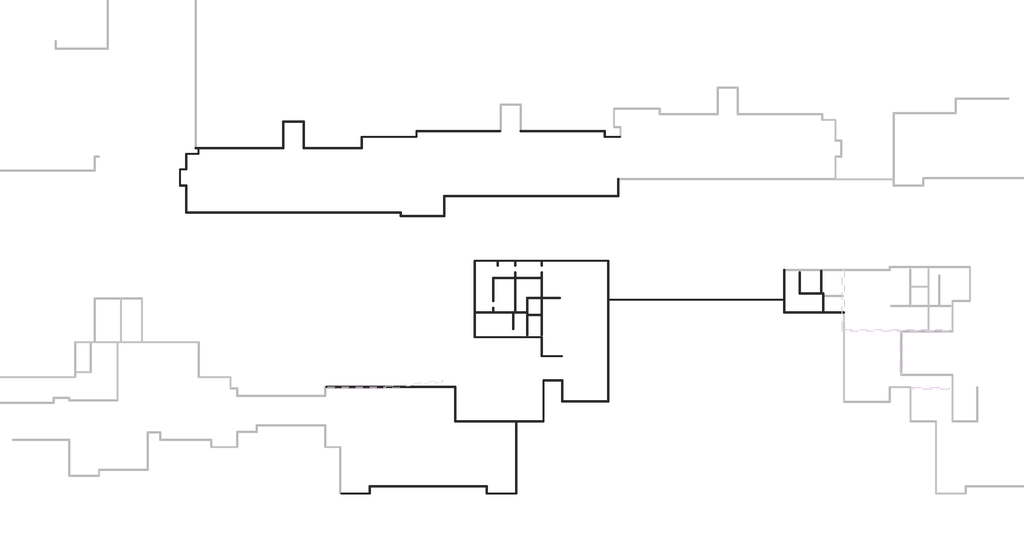
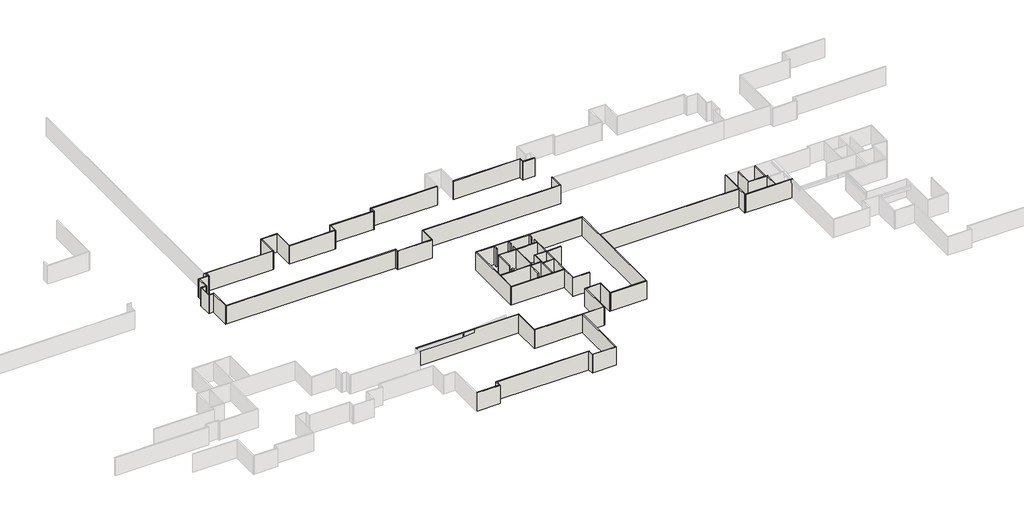
# One storey, part 4 of 8: 65 walls.
"""IFC4 building model written with IfcOpenShell, lengths in millimetres."""

from ifc_helpers import new_model, si_unit, origin, origin_with_axes, place, context, project, spatial, polyline, outline, extrude, faceted_brep, element, save

model = new_model("IFC4")

# Units and contexts
model_context = context("Model", 3, world=origin())
ifc_project = project(units=[si_unit("LENGTHUNIT", "METRE", prefix="MILLI")], contexts=[model_context])

# Site, building, storey
site = spatial("IfcSite", under=ifc_project)
building = spatial("IfcBuilding", under=site)
storey = spatial("IfcBuildingStorey", under=building, Name="户型图", Elevation=0.0)

# Walls
placement = place(None, origin())
element("IfcWall", 1, ObjectType="所有墙体", at=placement, inside=storey, context=model_context, shape_type="Brep", body=[
    faceted_brep([(190584.1761986, 13145.7645172, 0.0), (194584.1250491, 13145.7645172, 0.0), (194584.1250491, 13145.7645172, 3300.0), (190584.1761986, 13145.7645172, 3300.0), (190584.1761986, 13265.7645172, 0.0), (190584.1761986, 13265.7645172, 3300.0), (194464.1250491, 13265.7645172, 3300.0), (194584.1250491, 13265.7645172, 3300.0), (194584.1250491, 13265.7645172, 0.0), (194464.1250491, 13265.7645172, 0.0)], [[[0, 1, 2, 3]], [[4, 5, 6, 7, 8, 9]], [[1, 0, 4, 9, 8]], [[3, 2, 7, 6, 5]], [[0, 3, 5, 4]], [[2, 1, 8, 7]]]),
])
element("IfcWall", 2, ObjectType="所有墙体", at=placement, inside=storey, context=model_context, shape_type="Brep", body=[
    faceted_brep([(194584.1250491, 13265.7645172, 0.0), (194584.1250491, 14145.6242927, 0.0), (194584.1250491, 14265.6242927, 0.0), (194584.1250491, 14265.6242927, 3300.0), (194584.1250491, 14145.6242927, 3300.0), (194584.1250491, 13265.7645172, 3300.0), (194464.1250491, 13265.7645172, 0.0), (194464.1250491, 13265.7645172, 3300.0), (194464.1250491, 14265.6242927, 3300.0), (194464.1250491, 14265.6242927, 0.0)], [[[0, 1, 2, 3, 4, 5]], [[6, 7, 8, 9]], [[2, 1, 0, 6, 9]], [[5, 4, 3, 8, 7]], [[0, 5, 7, 6]], [[3, 2, 9, 8]]]),
])
element("IfcWall", 3, ObjectType="所有墙体", at=placement, inside=storey, context=model_context, shape_type="Brep", body=[
    faceted_brep([(194584.1250491, 14145.6242927, 0.0), (210264.1178879, 14145.6242927, 0.0), (210384.1178879, 14145.6242927, 0.0), (210384.1178879, 14145.6242927, 3300.0), (210264.1178879, 14145.6242927, 3300.0), (194584.1250491, 14145.6242927, 3300.0), (194584.1250491, 14265.6242927, 0.0), (194584.1250491, 14265.6242927, 3300.0), (210384.1178879, 14265.6242927, 3300.0), (210384.1178879, 14265.6242927, 0.0)], [[[0, 1, 2, 3, 4, 5]], [[6, 7, 8, 9]], [[2, 1, 0, 6, 9]], [[5, 4, 3, 8, 7]], [[0, 5, 7, 6]], [[3, 2, 9, 8]]]),
])
element("IfcWall", 4, ObjectType="所有墙体", at=placement, inside=storey, context=model_context, shape_type="Brep", body=[
    faceted_brep([(210264.1178879, 14145.6242927, 0.0), (210264.1178879, 13145.7645172, 0.0), (210264.1178879, 13145.7645172, 3300.0), (210264.1178879, 14145.6242927, 3300.0), (210384.1178879, 14145.6242927, 0.0), (210384.1178879, 14145.6242927, 3300.0), (210384.1178879, 13265.7645172, 3300.0), (210384.1178879, 13145.7645172, 3300.0), (210384.1178879, 13145.7645172, 0.0), (210384.1178879, 13265.7645172, 0.0)], [[[0, 1, 2, 3]], [[4, 5, 6, 7, 8, 9]], [[1, 0, 4, 9, 8]], [[3, 2, 7, 6, 5]], [[0, 3, 5, 4]], [[2, 1, 8, 7]]]),
])
element("IfcWall", 5, ObjectType="所有墙体", at=placement, inside=storey, context=model_context, shape_type="Brep", body=[
    faceted_brep([(210384.1178879, 13145.7645172, 0.0), (214384.1922923, 13145.7645172, 0.0), (214384.1922923, 13145.7645172, 3300.0), (210384.1178879, 13145.7645172, 3300.0), (210384.1178879, 13265.7645172, 0.0), (210384.1178879, 13265.7645172, 3300.0), (214264.1922923, 13265.7645172, 3300.0), (214384.1922923, 13265.7645172, 3300.0), (214384.1922923, 13265.7645172, 0.0), (214264.1922923, 13265.7645172, 0.0)], [[[0, 1, 2, 3]], [[4, 5, 6, 7, 8, 9]], [[1, 0, 4, 9, 8]], [[3, 2, 7, 6, 5]], [[0, 3, 5, 4]], [[2, 1, 8, 7]]]),
])
element("IfcWall", 6, ObjectType="所有墙体", at=placement, inside=storey, context=model_context, shape_type="SweptSolid", body=[
    extrude(outline(polyline([(214384.1922923, 22945.5527507), (214384.1922923, 13265.7645172), (214264.1922923, 13265.7645172), (214264.1922923, 22945.5527507), (214384.1922923, 22945.5527507)])), origin_with_axes(), (0.0, 0.0, 1.0), 3300.0),
])
element("IfcWall", 7, ObjectType="所有墙体", at=placement, inside=storey, context=model_context, shape_type="Brep", body=[
    faceted_brep([(218064.1922923, 22945.5527507, 0.0), (218064.1922923, 28456.6703435, 0.0), (218064.1922923, 28576.6703435, 0.0), (218064.1922923, 28576.6703435, 3300.0), (218064.1922923, 28456.6703435, 3300.0), (218064.1922923, 22945.5527507, 3300.0), (217944.1922923, 22945.5527507, 0.0), (217944.1922923, 22945.5527507, 3300.0), (217944.1922923, 23065.5527507, 3300.0), (217944.1922923, 28576.6703435, 3300.0), (217944.1922923, 28576.6703435, 0.0), (217944.1922923, 23065.5527507, 0.0)], [[[0, 1, 2, 3, 4, 5]], [[6, 7, 8, 9, 10, 11]], [[2, 1, 0, 6, 11, 10]], [[5, 4, 3, 9, 8, 7]], [[3, 2, 10, 9]], [[0, 5, 7, 6]]]),
])
element("IfcWall", 8, ObjectType="所有墙体", at=placement, inside=storey, context=model_context, shape_type="Brep", body=[
    faceted_brep([(218064.1922923, 28456.6703435, 0.0), (220514.3505603, 28456.6703435, 0.0), (220634.3505603, 28456.6703435, 0.0), (220634.3505603, 28456.6703435, 3300.0), (220514.3505603, 28456.6703435, 3300.0), (218064.1922923, 28456.6703435, 3300.0), (218064.1922923, 28576.6703435, 0.0), (218064.1922923, 28576.6703435, 3300.0), (220634.3505603, 28576.6703435, 3300.0), (220634.3505603, 28576.6703435, 0.0)], [[[0, 1, 2, 3, 4, 5]], [[6, 7, 8, 9]], [[2, 1, 0, 6, 9]], [[5, 4, 3, 8, 7]], [[0, 5, 7, 6]], [[3, 2, 9, 8]]]),
])
element("IfcWall", 9, ObjectType="所有墙体", at=placement, inside=storey, context=model_context, shape_type="Brep", body=[
    faceted_brep([(220514.3505603, 28456.6703435, 0.0), (220514.3505603, 25645.6713095, 0.0), (220514.3505603, 25645.6713095, 3300.0), (220514.3505603, 28456.6703435, 3300.0), (220634.3505603, 28456.6703435, 0.0), (220634.3505603, 28456.6703435, 3300.0), (220634.3505603, 25765.6713095, 3300.0), (220634.3505603, 25645.6713095, 3300.0), (220634.3505603, 25645.6713095, 0.0), (220634.3505603, 25765.6713095, 0.0)], [[[0, 1, 2, 3]], [[4, 5, 6, 7, 8, 9]], [[1, 0, 4, 9, 8]], [[3, 2, 7, 6, 5]], [[0, 3, 5, 4]], [[2, 1, 8, 7]]]),
])
element("IfcWall", 10, ObjectType="所有墙体", at=placement, inside=storey, context=model_context, shape_type="Brep", body=[
    faceted_brep([(220634.3505603, 25645.6713095, 0.0), (226833.8525836, 25645.6713095, 0.0), (226833.8525836, 25645.6713095, 3300.0), (220634.3505603, 25645.6713095, 3300.0), (220634.3505603, 25765.6713095, 0.0), (220634.3505603, 25765.6713095, 3300.0), (226713.8525836, 25765.6713095, 3300.0), (226833.8525836, 25765.6713095, 3300.0), (226833.8525836, 25765.6713095, 0.0), (226713.8525836, 25765.6713095, 0.0)], [[[0, 1, 2, 3]], [[4, 5, 6, 7, 8, 9]], [[1, 0, 4, 9, 8]], [[3, 2, 7, 6, 5]], [[0, 3, 5, 4]], [[2, 1, 8, 7]]]),
])
element("IfcWall", 11, ObjectType="所有墙体", at=placement, inside=storey, context=model_context, shape_type="Brep", body=[
    faceted_brep([(226833.8525836, 25765.6713095, 0.0), (226833.8525836, 39406.3533948, 0.0), (226833.8525836, 39526.3533948, 0.0), (226833.8525836, 44681.8474602, 0.0), (226833.8525836, 44681.8474602, 3300.0), (226833.8525836, 39526.3533948, 3300.0), (226833.8525836, 39406.3533948, 3300.0), (226833.8525836, 25765.6713095, 3300.0), (226713.8525836, 25765.6713095, 0.0), (226713.8525836, 25765.6713095, 3300.0), (226713.8525836, 44681.8474602, 3300.0), (226713.8525836, 44681.8474602, 0.0)], [[[0, 1, 2, 3, 4, 5, 6, 7]], [[8, 9, 10, 11]], [[3, 2, 1, 0, 8, 11]], [[7, 6, 5, 4, 10, 9]], [[0, 7, 9, 8]], [[4, 3, 11, 10]]]),
])
element("IfcWall", 12, ObjectType="所有墙体", at=placement, inside=storey, context=model_context, shape_type="SweptSolid", body=[
    extrude(outline(polyline([(250538.8239575, 39406.3533948), (226833.8525836, 39406.3533948), (226833.8525836, 39526.3533948), (250538.8239575, 39526.3533948), (250538.8239575, 39406.3533948)])), origin_with_axes(), (0.0, 0.0, 1.0), 3300.0),
])
element("IfcWall", 13, ObjectType="所有墙体", at=placement, inside=storey, context=model_context, shape_type="Brep", body=[
    faceted_brep([(250538.8239575, 43526.8473728, 0.0), (250538.8239575, 39526.3533948, 0.0), (250538.8239575, 39406.3533948, 0.0), (250538.8239575, 37656.7427445, 0.0), (250538.8239575, 37656.7427445, 3300.0), (250538.8239575, 39406.3533948, 3300.0), (250538.8239575, 39526.3533948, 3300.0), (250538.8239575, 43526.8473728, 3300.0), (250658.8239575, 43526.8473728, 0.0), (250658.8239575, 43526.8473728, 3300.0), (250658.8239575, 43406.8473728, 3300.0), (250658.8239575, 37776.7427445, 3300.0), (250658.8239575, 37656.7427445, 3300.0), (250658.8239575, 37656.7427445, 0.0), (250658.8239575, 37776.7427445, 0.0), (250658.8239575, 43406.8473728, 0.0)], [[[0, 1, 2, 3, 4, 5, 6, 7]], [[8, 9, 10, 11, 12, 13, 14, 15]], [[3, 2, 1, 0, 8, 15, 14, 13]], [[7, 6, 5, 4, 12, 11, 10, 9]], [[4, 3, 13, 12]], [[0, 7, 9, 8]]]),
])
element("IfcWall", 14, ObjectType="所有墙体", at=placement, inside=storey, context=model_context, shape_type="Brep", body=[
    faceted_brep([(250658.8239575, 37656.7427445, 0.0), (258613.8534901, 37656.7427445, 0.0), (258733.8534901, 37656.7427445, 0.0), (258733.8534901, 37656.7427445, 3300.0), (258613.8534901, 37656.7427445, 3300.0), (250658.8239575, 37656.7427445, 3300.0), (250658.8239575, 37776.7427445, 0.0), (250658.8239575, 37776.7427445, 3300.0), (255788.6559976, 37776.7427445, 3300.0), (255908.6559976, 37776.7427445, 3300.0), (258733.8534901, 37776.7427445, 3300.0), (258733.8534901, 37776.7427445, 0.0), (255908.6559976, 37776.7427445, 0.0), (255788.6559976, 37776.7427445, 0.0)], [[[0, 1, 2, 3, 4, 5]], [[6, 7, 8, 9, 10, 11, 12, 13]], [[2, 1, 0, 6, 13, 12, 11]], [[5, 4, 3, 10, 9, 8, 7]], [[0, 5, 7, 6]], [[3, 2, 11, 10]]]),
])
element("IfcWall", 15, ObjectType="所有墙体", at=placement, inside=storey, context=model_context, shape_type="Brep", body=[
    faceted_brep([(228364.4881621, 61576.5107166, 0.0), (226384.4923674, 61576.5107166, 0.0), (226264.4923674, 61576.5107166, 0.0), (226264.4923674, 61576.5107166, 3300.0), (226384.4923674, 61576.5107166, 3300.0), (228364.4881621, 61576.5107166, 3300.0), (228364.4881621, 61456.5107166, 0.0), (228364.4881621, 61456.5107166, 3300.0), (226264.4923674, 61456.5107166, 3300.0), (226264.4923674, 61456.5107166, 0.0)], [[[0, 1, 2, 3, 4, 5]], [[6, 7, 8, 9]], [[2, 1, 0, 6, 9]], [[5, 4, 3, 8, 7]], [[0, 5, 7, 6]], [[3, 2, 9, 8]]]),
])
element("IfcWall", 16, ObjectType="所有墙体", at=placement, inside=storey, context=model_context, shape_type="Brep", body=[
    faceted_brep([(226384.4923674, 61576.5107166, 0.0), (226384.4923674, 62376.635741, 0.0), (226384.4923674, 62376.635741, 3300.0), (226384.4923674, 61576.5107166, 3300.0), (226264.4923674, 61576.5107166, 0.0), (226264.4923674, 61576.5107166, 3300.0), (226264.4923674, 62256.635741, 3300.0), (226264.4923674, 62376.635741, 3300.0), (226264.4923674, 62376.635741, 0.0), (226264.4923674, 62256.635741, 0.0)], [[[0, 1, 2, 3]], [[4, 5, 6, 7, 8, 9]], [[1, 0, 4, 9, 8]], [[3, 2, 7, 6, 5]], [[0, 3, 5, 4]], [[2, 1, 8, 7]]]),
])
element("IfcWall", 17, ObjectType="所有墙体", at=placement, inside=storey, context=model_context, shape_type="Brep", body=[
    faceted_brep([(226264.4923674, 62376.635741, 0.0), (214984.4914101, 62376.635741, 0.0), (214864.4914101, 62376.635741, 0.0), (214864.4914101, 62376.635741, 3300.0), (214984.4914101, 62376.635741, 3300.0), (226264.4923674, 62376.635741, 3300.0), (226264.4923674, 62256.635741, 0.0), (226264.4923674, 62256.635741, 3300.0), (214864.4914101, 62256.635741, 3300.0), (214864.4914101, 62256.635741, 0.0)], [[[0, 1, 2, 3, 4, 5]], [[6, 7, 8, 9]], [[2, 1, 0, 6, 9]], [[5, 4, 3, 8, 7]], [[0, 5, 7, 6]], [[3, 2, 9, 8]]]),
])
element("IfcWall", 18, ObjectType="所有墙体", at=placement, inside=storey, context=model_context, shape_type="Brep", body=[
    faceted_brep([(212164.4916662, 62376.635741, 0.0), (200764.4747442, 62376.635741, 0.0), (200764.4747442, 62376.635741, 3300.0), (212164.4916662, 62376.635741, 3300.0), (212164.4916662, 62256.635741, 0.0), (212164.4916662, 62256.635741, 3300.0), (200884.4747442, 62256.635741, 3300.0), (200764.4747442, 62256.635741, 3300.0), (200764.4747442, 62256.635741, 0.0), (200884.4747442, 62256.635741, 0.0)], [[[0, 1, 2, 3]], [[4, 5, 6, 7, 8, 9]], [[1, 0, 4, 9, 8]], [[3, 2, 7, 6, 5]], [[0, 3, 5, 4]], [[2, 1, 8, 7]]]),
])
element("IfcWall", 19, ObjectType="所有墙体", at=placement, inside=storey, context=model_context, shape_type="Brep", body=[
    faceted_brep([(200764.4747442, 62256.635741, 0.0), (200764.4747442, 61576.5107166, 0.0), (200764.4747442, 61456.5107166, 0.0), (200764.4747442, 61456.5107166, 3300.0), (200764.4747442, 61576.5107166, 3300.0), (200764.4747442, 62256.635741, 3300.0), (200884.4747442, 62256.635741, 0.0), (200884.4747442, 62256.635741, 3300.0), (200884.4747442, 61456.5107166, 3300.0), (200884.4747442, 61456.5107166, 0.0)], [[[0, 1, 2, 3, 4, 5]], [[6, 7, 8, 9]], [[2, 1, 0, 6, 9]], [[5, 4, 3, 8, 7]], [[0, 5, 7, 6]], [[3, 2, 9, 8]]]),
])
element("IfcWall", 20, ObjectType="所有墙体", at=placement, inside=storey, context=model_context, shape_type="Brep", body=[
    faceted_brep([(200764.4747442, 61576.5107166, 0.0), (193364.4739968, 61576.5107166, 0.0), (193364.4739968, 61576.5107166, 3300.0), (200764.4747442, 61576.5107166, 3300.0), (200764.4747442, 61456.5107166, 0.0), (200764.4747442, 61456.5107166, 3300.0), (193484.4739968, 61456.5107166, 3300.0), (193364.4739968, 61456.5107166, 3300.0), (193364.4739968, 61456.5107166, 0.0), (193484.4739968, 61456.5107166, 0.0)], [[[0, 1, 2, 3]], [[4, 5, 6, 7, 8, 9]], [[1, 0, 4, 9, 8]], [[3, 2, 7, 6, 5]], [[0, 3, 5, 4]], [[2, 1, 8, 7]]]),
])
element("IfcWall", 21, ObjectType="所有墙体", at=placement, inside=storey, context=model_context, shape_type="Brep", body=[
    faceted_brep([(193364.4739968, 61456.5107166, 0.0), (193364.4739968, 60076.635667, 0.0), (193364.4739968, 59956.635667, 0.0), (193364.4739968, 59956.635667, 3300.0), (193364.4739968, 60076.635667, 3300.0), (193364.4739968, 61456.5107166, 3300.0), (193484.4739968, 61456.5107166, 0.0), (193484.4739968, 61456.5107166, 3300.0), (193484.4739968, 59956.635667, 3300.0), (193484.4739968, 59956.635667, 0.0)], [[[0, 1, 2, 3, 4, 5]], [[6, 7, 8, 9]], [[2, 1, 0, 6, 9]], [[5, 4, 3, 8, 7]], [[0, 5, 7, 6]], [[3, 2, 9, 8]]]),
])
element("IfcWall", 22, ObjectType="所有墙体", at=placement, inside=storey, context=model_context, shape_type="Brep", body=[
    faceted_brep([(193364.4739968, 60076.635667, 0.0), (185609.4693749, 60076.635667, 0.0), (185489.4693749, 60076.635667, 0.0), (185489.4693749, 60076.635667, 3300.0), (185609.4693749, 60076.635667, 3300.0), (193364.4739968, 60076.635667, 3300.0), (193364.4739968, 59956.635667, 0.0), (193364.4739968, 59956.635667, 3300.0), (185489.4693749, 59956.635667, 3300.0), (185489.4693749, 59956.635667, 0.0)], [[[0, 1, 2, 3, 4, 5]], [[6, 7, 8, 9]], [[2, 1, 0, 6, 9]], [[5, 4, 3, 8, 7]], [[0, 5, 7, 6]], [[3, 2, 9, 8]]]),
])
element("IfcWall", 23, ObjectType="所有墙体", at=placement, inside=storey, context=model_context, shape_type="Brep", body=[
    faceted_brep([(185609.4693749, 60076.635667, 0.0), (185609.4693749, 63651.6355965, 0.0), (185609.4693749, 63651.6355965, 3300.0), (185609.4693749, 60076.635667, 3300.0), (185489.4693749, 60076.635667, 0.0), (185489.4693749, 60076.635667, 3300.0), (185489.4693749, 63531.6355965, 3300.0), (185489.4693749, 63651.6355965, 3300.0), (185489.4693749, 63651.6355965, 0.0), (185489.4693749, 63531.6355965, 0.0)], [[[0, 1, 2, 3]], [[4, 5, 6, 7, 8, 9]], [[1, 0, 4, 9, 8]], [[3, 2, 7, 6, 5]], [[0, 3, 5, 4]], [[2, 1, 8, 7]]]),
])
element("IfcWall", 24, ObjectType="所有墙体", at=placement, inside=storey, context=model_context, shape_type="Brep", body=[
    faceted_brep([(185489.4693749, 63651.6355965, 0.0), (182739.4693749, 63651.6355965, 0.0), (182739.4693749, 63651.6355965, 3300.0), (185489.4693749, 63651.6355965, 3300.0), (185489.4693749, 63531.6355965, 0.0), (185489.4693749, 63531.6355965, 3300.0), (182859.4693749, 63531.6355965, 3300.0), (182739.4693749, 63531.6355965, 3300.0), (182739.4693749, 63531.6355965, 0.0), (182859.4693749, 63531.6355965, 0.0)], [[[0, 1, 2, 3]], [[4, 5, 6, 7, 8, 9]], [[1, 0, 4, 9, 8]], [[3, 2, 7, 6, 5]], [[0, 3, 5, 4]], [[2, 1, 8, 7]]]),
])
element("IfcWall", 25, ObjectType="所有墙体", at=placement, inside=storey, context=model_context, shape_type="Brep", body=[
    faceted_brep([(182739.4693749, 63531.6355965, 0.0), (182739.4693749, 60076.635667, 0.0), (182739.4693749, 59956.635667, 0.0), (182739.4693749, 59956.635667, 3300.0), (182739.4693749, 60076.635667, 3300.0), (182739.4693749, 63531.6355965, 3300.0), (182859.4693749, 63531.6355965, 0.0), (182859.4693749, 63531.6355965, 3300.0), (182859.4693749, 59956.635667, 3300.0), (182859.4693749, 59956.635667, 0.0)], [[[0, 1, 2, 3, 4, 5]], [[6, 7, 8, 9]], [[2, 1, 0, 6, 9]], [[5, 4, 3, 8, 7]], [[0, 5, 7, 6]], [[3, 2, 9, 8]]]),
])
element("IfcWall", 26, ObjectType="所有墙体", at=placement, inside=storey, context=model_context, shape_type="Brep", body=[
    faceted_brep([(182739.4693749, 60076.635667, 0.0), (171033.8238906, 60076.635667, 0.0), (170913.8238906, 60076.635667, 0.0), (170913.8238906, 60076.635667, 3300.0), (171033.8238906, 60076.635667, 3300.0), (182739.4693749, 60076.635667, 3300.0), (182739.4693749, 59956.635667, 0.0), (182739.4693749, 59956.635667, 3300.0), (171384.4744322, 59956.635667, 3300.0), (171264.4744322, 59956.635667, 3300.0), (170913.8238906, 59956.635667, 3300.0), (170913.8238906, 59956.635667, 0.0), (171264.4744322, 59956.635667, 0.0), (171384.4744322, 59956.635667, 0.0)], [[[0, 1, 2, 3, 4, 5]], [[6, 7, 8, 9, 10, 11, 12, 13]], [[2, 1, 0, 6, 13, 12, 11]], [[5, 4, 3, 10, 9, 8, 7]], [[0, 5, 7, 6]], [[3, 2, 11, 10]]]),
])
element("IfcWall", 27, ObjectType="所有墙体", at=placement, inside=storey, context=model_context, shape_type="Brep", body=[
    faceted_brep([(188533.8473665, 27606.8378863, 0.0), (206001.3464068, 27606.8378863, 0.0), (206121.3464068, 27606.8378863, 0.0), (206121.3464068, 27606.8378863, 3300.0), (206001.3464068, 27606.8378863, 3300.0), (188533.8473665, 27606.8378863, 3300.0), (188533.8473665, 27726.8378863, 0.0), (188533.8473665, 27726.8378863, 3300.0), (206121.3464068, 27726.8378863, 3300.0), (206121.3464068, 27726.8378863, 0.0)], [[[0, 1, 2, 3, 4, 5]], [[6, 7, 8, 9]], [[2, 1, 0, 6, 9]], [[5, 4, 3, 8, 7]], [[0, 5, 7, 6]], [[3, 2, 9, 8]]]),
])
element("IfcWall", 28, ObjectType="所有墙体", at=placement, inside=storey, context=model_context, shape_type="Brep", body=[
    faceted_brep([(206001.3464068, 27606.8378863, 0.0), (206001.3464068, 22945.5527507, 0.0), (206001.3464068, 22945.5527507, 3300.0), (206001.3464068, 27606.8378863, 3300.0), (206121.3464068, 27606.8378863, 0.0), (206121.3464068, 27606.8378863, 3300.0), (206121.3464068, 23065.5527507, 3300.0), (206121.3464068, 22945.5527507, 3300.0), (206121.3464068, 22945.5527507, 0.0), (206121.3464068, 23065.5527507, 0.0)], [[[0, 1, 2, 3]], [[4, 5, 6, 7, 8, 9]], [[1, 0, 4, 9, 8]], [[3, 2, 7, 6, 5]], [[0, 3, 5, 4]], [[2, 1, 8, 7]]]),
])
element("IfcWall", 29, ObjectType="所有墙体", at=placement, inside=storey, context=model_context, shape_type="Brep", body=[
    faceted_brep([(206121.3464068, 22945.5527507, 0.0), (214264.1922923, 22945.5527507, 0.0), (214384.1922923, 22945.5527507, 0.0), (217944.1922923, 22945.5527507, 0.0), (217944.1922923, 22945.5527507, 3300.0), (214384.1922923, 22945.5527507, 3300.0), (214264.1922923, 22945.5527507, 3300.0), (206121.3464068, 22945.5527507, 3300.0), (206121.3464068, 23065.5527507, 0.0), (206121.3464068, 23065.5527507, 3300.0), (217944.1922923, 23065.5527507, 3300.0), (217944.1922923, 23065.5527507, 0.0)], [[[0, 1, 2, 3, 4, 5, 6, 7]], [[8, 9, 10, 11]], [[3, 2, 1, 0, 8, 11]], [[7, 6, 5, 4, 10, 9]], [[0, 7, 9, 8]], [[4, 3, 11, 10]]]),
])
element("IfcWall", 30, ObjectType="所有墙体", at=placement, inside=storey, context=model_context, shape_type="Brep", body=[
    faceted_brep([(171264.4744322, 59956.635667, 0.0), (171264.4744322, 59276.635667, 0.0), (171264.4744322, 59156.635667, 0.0), (171264.4744322, 59156.635667, 3300.0), (171264.4744322, 59276.635667, 3300.0), (171264.4744322, 59956.635667, 3300.0), (171384.4744322, 59956.635667, 0.0), (171384.4744322, 59956.635667, 3300.0), (171384.4744322, 59156.635667, 3300.0), (171384.4744322, 59156.635667, 0.0)], [[[0, 1, 2, 3, 4, 5]], [[6, 7, 8, 9]], [[2, 1, 0, 6, 9]], [[5, 4, 3, 8, 7]], [[0, 5, 7, 6]], [[3, 2, 9, 8]]]),
])
element("IfcWall", 31, ObjectType="所有墙体", at=placement, inside=storey, context=model_context, shape_type="Brep", body=[
    faceted_brep([(171264.4744322, 59276.635667, 0.0), (169589.4656792, 59276.635667, 0.0), (169589.4656792, 59276.635667, 3300.0), (171264.4744322, 59276.635667, 3300.0), (171264.4744322, 59156.635667, 0.0), (171264.4744322, 59156.635667, 3300.0), (169709.4656792, 59156.635667, 3300.0), (169589.4656792, 59156.635667, 3300.0), (169589.4656792, 59156.635667, 0.0), (169709.4656792, 59156.635667, 0.0)], [[[0, 1, 2, 3]], [[4, 5, 6, 7, 8, 9]], [[1, 0, 4, 9, 8]], [[3, 2, 7, 6, 5]], [[0, 3, 5, 4]], [[2, 1, 8, 7]]]),
])
element("IfcWall", 32, ObjectType="所有墙体", at=placement, inside=storey, context=model_context, shape_type="Brep", body=[
    faceted_brep([(169589.4656792, 59156.635667, 0.0), (169589.4656792, 57176.6357317, 0.0), (169589.4656792, 57056.6357317, 0.0), (169589.4656792, 57056.6357317, 3300.0), (169589.4656792, 57176.6357317, 3300.0), (169589.4656792, 59156.635667, 3300.0), (169709.4656792, 59156.635667, 0.0), (169709.4656792, 59156.635667, 3300.0), (169709.4656792, 57056.6357317, 3300.0), (169709.4656792, 57056.6357317, 0.0)], [[[0, 1, 2, 3, 4, 5]], [[6, 7, 8, 9]], [[2, 1, 0, 6, 9]], [[5, 4, 3, 8, 7]], [[0, 5, 7, 6]], [[3, 2, 9, 8]]]),
])
element("IfcWall", 33, ObjectType="所有墙体", at=placement, inside=storey, context=model_context, shape_type="Brep", body=[
    faceted_brep([(169589.4656792, 57176.6357317, 0.0), (168764.4909106, 57176.6357317, 0.0), (168764.4909106, 57176.6357317, 3300.0), (169589.4656792, 57176.6357317, 3300.0), (169589.4656792, 57056.6357317, 0.0), (169589.4656792, 57056.6357317, 3300.0), (168884.4909106, 57056.6357317, 3300.0), (168764.4909106, 57056.6357317, 3300.0), (168764.4909106, 57056.6357317, 0.0), (168884.4909106, 57056.6357317, 0.0)], [[[0, 1, 2, 3]], [[4, 5, 6, 7, 8, 9]], [[1, 0, 4, 9, 8]], [[3, 2, 7, 6, 5]], [[0, 3, 5, 4]], [[2, 1, 8, 7]]]),
])
element("IfcWall", 34, ObjectType="所有墙体", at=placement, inside=storey, context=model_context, shape_type="Brep", body=[
    faceted_brep([(168764.4909106, 57056.6357317, 0.0), (168764.4909106, 54856.6356701, 0.0), (168764.4909106, 54856.6356701, 3300.0), (168764.4909106, 57056.6357317, 3300.0), (168884.4909106, 57056.6357317, 0.0), (168884.4909106, 57056.6357317, 3300.0), (168884.4909106, 54976.6356701, 3300.0), (168884.4909106, 54856.6356701, 3300.0), (168884.4909106, 54856.6356701, 0.0), (168884.4909106, 54976.6356701, 0.0)], [[[0, 1, 2, 3]], [[4, 5, 6, 7, 8, 9]], [[1, 0, 4, 9, 8]], [[3, 2, 7, 6, 5]], [[0, 3, 5, 4]], [[2, 1, 8, 7]]]),
])
element("IfcWall", 35, ObjectType="所有墙体", at=placement, inside=storey, context=model_context, shape_type="Brep", body=[
    faceted_brep([(168884.4909106, 54856.6356701, 0.0), (169589.4656792, 54856.6356701, 0.0), (169709.4656792, 54856.6356701, 0.0), (169709.4656792, 54856.6356701, 3300.0), (169589.4656792, 54856.6356701, 3300.0), (168884.4909106, 54856.6356701, 3300.0), (168884.4909106, 54976.6356701, 0.0), (168884.4909106, 54976.6356701, 3300.0), (169709.4656792, 54976.6356701, 3300.0), (169709.4656792, 54976.6356701, 0.0)], [[[0, 1, 2, 3, 4, 5]], [[6, 7, 8, 9]], [[2, 1, 0, 6, 9]], [[5, 4, 3, 8, 7]], [[0, 5, 7, 6]], [[3, 2, 9, 8]]]),
])
element("IfcWall", 36, ObjectType="所有墙体", at=placement, inside=storey, context=model_context, shape_type="Brep", body=[
    faceted_brep([(169589.4656792, 54856.6356701, 0.0), (169589.4656792, 51181.636538, 0.0), (169589.4656792, 51181.636538, 3300.0), (169589.4656792, 54856.6356701, 3300.0), (169709.4656792, 54856.6356701, 0.0), (169709.4656792, 54856.6356701, 3300.0), (169709.4656792, 51301.636538, 3300.0), (169709.4656792, 51181.636538, 3300.0), (169709.4656792, 51181.636538, 0.0), (169709.4656792, 51301.636538, 0.0)], [[[0, 1, 2, 3]], [[4, 5, 6, 7, 8, 9]], [[1, 0, 4, 9, 8]], [[3, 2, 7, 6, 5]], [[0, 3, 5, 4]], [[2, 1, 8, 7]]]),
])
element("IfcWall", 37, ObjectType="所有墙体", at=placement, inside=storey, context=model_context, shape_type="Brep", body=[
    faceted_brep([(169709.4656792, 51181.636538, 0.0), (198639.2539647, 51181.636538, 0.0), (198759.2539647, 51181.636538, 0.0), (198759.2539647, 51181.636538, 3300.0), (198639.2539647, 51181.636538, 3300.0), (169709.4656792, 51181.636538, 3300.0), (169709.4656792, 51301.636538, 0.0), (169709.4656792, 51301.636538, 3300.0), (198759.2539647, 51301.636538, 3300.0), (198759.2539647, 51301.636538, 0.0)], [[[0, 1, 2, 3, 4, 5]], [[6, 7, 8, 9]], [[2, 1, 0, 6, 9]], [[5, 4, 3, 8, 7]], [[0, 5, 7, 6]], [[3, 2, 9, 8]]]),
])
element("IfcWall", 38, ObjectType="所有墙体", at=placement, inside=storey, context=model_context, shape_type="Brep", body=[
    faceted_brep([(198639.2539647, 51181.636538, 0.0), (198639.2539647, 50706.7424842, 0.0), (198639.2539647, 50706.7424842, 3300.0), (198639.2539647, 51181.636538, 3300.0), (198759.2539647, 51181.636538, 0.0), (198759.2539647, 51181.636538, 3300.0), (198759.2539647, 50826.7424842, 3300.0), (198759.2539647, 50706.7424842, 3300.0), (198759.2539647, 50706.7424842, 0.0), (198759.2539647, 50826.7424842, 0.0)], [[[0, 1, 2, 3]], [[4, 5, 6, 7, 8, 9]], [[1, 0, 4, 9, 8]], [[3, 2, 7, 6, 5]], [[0, 3, 5, 4]], [[2, 1, 8, 7]]]),
])
element("IfcWall", 39, ObjectType="所有墙体", at=placement, inside=storey, context=model_context, shape_type="Brep", body=[
    faceted_brep([(198759.2539647, 50706.7424842, 0.0), (204658.835888, 50706.7424842, 0.0), (204658.835888, 50706.7424842, 3300.0), (198759.2539647, 50706.7424842, 3300.0), (198759.2539647, 50826.7424842, 0.0), (198759.2539647, 50826.7424842, 3300.0), (204538.835888, 50826.7424842, 3300.0), (204658.835888, 50826.7424842, 3300.0), (204658.835888, 50826.7424842, 0.0), (204538.835888, 50826.7424842, 0.0)], [[[0, 1, 2, 3]], [[4, 5, 6, 7, 8, 9]], [[1, 0, 4, 9, 8]], [[3, 2, 7, 6, 5]], [[0, 3, 5, 4]], [[2, 1, 8, 7]]]),
])
element("IfcWall", 40, ObjectType="所有墙体", at=placement, inside=storey, context=model_context, shape_type="Brep", body=[
    faceted_brep([(204658.835888, 50826.7424842, 0.0), (204658.835888, 53456.6355075, 0.0), (204658.835888, 53576.6355075, 0.0), (204658.835888, 53576.6355075, 3300.0), (204658.835888, 53456.6355075, 3300.0), (204658.835888, 50826.7424842, 3300.0), (204538.835888, 50826.7424842, 0.0), (204538.835888, 50826.7424842, 3300.0), (204538.835888, 53576.6355075, 3300.0), (204538.835888, 53576.6355075, 0.0)], [[[0, 1, 2, 3, 4, 5]], [[6, 7, 8, 9]], [[2, 1, 0, 6, 9]], [[5, 4, 3, 8, 7]], [[0, 5, 7, 6]], [[3, 2, 9, 8]]]),
])
element("IfcWall", 41, ObjectType="所有墙体", at=placement, inside=storey, context=model_context, shape_type="Brep", body=[
    faceted_brep([(204658.835888, 53456.6355075, 0.0), (228184.5003905, 53456.6355075, 0.0), (228184.5003905, 53456.6355075, 3300.0), (204658.835888, 53456.6355075, 3300.0), (204658.835888, 53576.6355075, 0.0), (204658.835888, 53576.6355075, 3300.0), (228064.5003905, 53576.6355075, 3300.0), (228184.5003905, 53576.6355075, 3300.0), (228184.5003905, 53576.6355075, 0.0), (228064.5003905, 53576.6355075, 0.0)], [[[0, 1, 2, 3]], [[4, 5, 6, 7, 8, 9]], [[1, 0, 4, 9, 8]], [[3, 2, 7, 6, 5]], [[0, 3, 5, 4]], [[2, 1, 8, 7]]]),
])
element("IfcWall", 42, ObjectType="所有墙体", at=placement, inside=storey, context=model_context, shape_type="Brep", body=[
    faceted_brep([(228184.5003905, 53576.6355075, 0.0), (228184.5003905, 55756.5110329, 0.0), (228184.5003905, 55876.5110329, 0.0), (228184.5003905, 55876.5110329, 3300.0), (228184.5003905, 55756.5110329, 3300.0), (228184.5003905, 53576.6355075, 3300.0), (228064.5003905, 53576.6355075, 0.0), (228064.5003905, 53576.6355075, 3300.0), (228064.5003905, 55876.5110329, 3300.0), (228064.5003905, 55876.5110329, 0.0)], [[[0, 1, 2, 3, 4, 5]], [[6, 7, 8, 9]], [[2, 1, 0, 6, 9]], [[5, 4, 3, 8, 7]], [[0, 5, 7, 6]], [[3, 2, 9, 8]]]),
])
element("IfcWall", 43, ObjectType="所有墙体", at=placement, inside=storey, context=model_context, shape_type="Brep", body=[
    faceted_brep([(220574.3505603, 31876.9409691, 0.0), (217859.3835375, 31876.9409691, 0.0), (217739.3835375, 31876.9409691, 0.0), (217739.3835375, 31876.9409691, 3300.0), (217859.3835375, 31876.9409691, 3300.0), (220574.3505603, 31876.9409691, 3300.0), (220574.3505603, 31756.9409691, 0.0), (220574.3505603, 31756.9409691, 3300.0), (217739.3835375, 31756.9409691, 3300.0), (217739.3835375, 31756.9409691, 0.0)], [[[0, 1, 2, 3, 4, 5]], [[6, 7, 8, 9]], [[2, 1, 0, 6, 9]], [[5, 4, 3, 8, 7]], [[0, 5, 7, 6]], [[3, 2, 9, 8]]]),
])
element("IfcWall", 44, ObjectType="所有墙体", at=placement, inside=storey, context=model_context, shape_type="Brep", body=[
    faceted_brep([(217859.3835375, 31876.9409691, 0.0), (217859.3835375, 34451.846369, 0.0), (217859.3835375, 34451.846369, 3300.0), (217859.3835375, 31876.9409691, 3300.0), (217739.3835375, 31876.9409691, 0.0), (217739.3835375, 31876.9409691, 3300.0), (217739.3835375, 34331.846369, 3300.0), (217739.3835375, 34451.846369, 3300.0), (217739.3835375, 34451.846369, 0.0), (217739.3835375, 34331.846369, 0.0)], [[[0, 1, 2, 3]], [[4, 5, 6, 7, 8, 9]], [[1, 0, 4, 9, 8]], [[3, 2, 7, 6, 5]], [[0, 3, 5, 4]], [[2, 1, 8, 7]]]),
])
element("IfcWall", 45, ObjectType="所有墙体", at=placement, inside=storey, context=model_context, shape_type="Brep", body=[
    faceted_brep([(217739.3835375, 34451.846369, 0.0), (208783.8790441, 34451.846369, 0.0), (208663.8790441, 34451.846369, 0.0), (208663.8790441, 34451.846369, 3300.0), (208783.8790441, 34451.846369, 3300.0), (217739.3835375, 34451.846369, 3300.0), (217739.3835375, 34331.846369, 0.0), (217739.3835375, 34331.846369, 3300.0), (208663.8790441, 34331.846369, 3300.0), (208663.8790441, 34331.846369, 0.0)], [[[0, 1, 2, 3, 4, 5]], [[6, 7, 8, 9]], [[2, 1, 0, 6, 9]], [[5, 4, 3, 8, 7]], [[0, 5, 7, 6]], [[3, 2, 9, 8]]]),
])
element("IfcWall", 46, ObjectType="所有墙体", at=placement, inside=storey, context=model_context, shape_type="Brep", body=[
    faceted_brep([(208783.8790441, 34451.846369, 0.0), (208783.8790441, 37691.846369, 0.0), (208783.8790441, 37811.846369, 0.0), (208783.8790441, 44681.8474602, 0.0), (208783.8790441, 44801.8474602, 0.0), (208783.8790441, 44801.8474602, 3300.0), (208783.8790441, 44681.8474602, 3300.0), (208783.8790441, 37811.846369, 3300.0), (208783.8790441, 37691.846369, 3300.0), (208783.8790441, 34451.846369, 3300.0), (208663.8790441, 34451.846369, 0.0), (208663.8790441, 34451.846369, 3300.0), (208663.8790441, 44801.8474602, 3300.0), (208663.8790441, 44801.8474602, 0.0)], [[[0, 1, 2, 3, 4, 5, 6, 7, 8, 9]], [[10, 11, 12, 13]], [[4, 3, 2, 1, 0, 10, 13]], [[9, 8, 7, 6, 5, 12, 11]], [[0, 9, 11, 10]], [[5, 4, 13, 12]]]),
])
element("IfcWall", 47, ObjectType="所有墙体", at=placement, inside=storey, context=model_context, shape_type="Brep", body=[
    faceted_brep([(208783.8790441, 44681.8474602, 0.0), (211739.1749325, 44681.8474602, 0.0), (211859.1749325, 44681.8474602, 0.0), (214124.2829345, 44681.8474602, 0.0), (214244.2829345, 44681.8474602, 0.0), (217688.8658138, 44681.8474602, 0.0), (217808.8658138, 44681.8474602, 0.0), (226713.8525836, 44681.8474602, 0.0), (226833.8525836, 44681.8474602, 0.0), (226833.8525836, 44681.8474602, 3300.0), (226713.8525836, 44681.8474602, 3300.0), (217808.8658138, 44681.8474602, 3300.0), (217688.8658138, 44681.8474602, 3300.0), (214244.2829345, 44681.8474602, 3300.0), (214124.2829345, 44681.8474602, 3300.0), (211859.1749325, 44681.8474602, 3300.0), (211739.1749325, 44681.8474602, 3300.0), (208783.8790441, 44681.8474602, 3300.0), (208783.8790441, 44801.8474602, 0.0), (208783.8790441, 44801.8474602, 3300.0), (226833.8525836, 44801.8474602, 3300.0), (226833.8525836, 44801.8474602, 0.0)], [[[0, 1, 2, 3, 4, 5, 6, 7, 8, 9, 10, 11, 12, 13, 14, 15, 16, 17]], [[18, 19, 20, 21]], [[8, 7, 6, 5, 4, 3, 2, 1, 0, 18, 21]], [[17, 16, 15, 14, 13, 12, 11, 10, 9, 20, 19]], [[0, 17, 19, 18]], [[9, 8, 21, 20]]]),
])
element("IfcWall", 48, ObjectType="所有墙体", at=placement, inside=storey, context=model_context, shape_type="Brep", body=[
    faceted_brep([(208783.8790441, 37691.846369, 0.0), (213864.2829345, 37691.846369, 0.0), (213984.2829345, 37691.846369, 0.0), (215739.2821437, 37691.846369, 0.0), (215739.2821437, 37691.846369, 3300.0), (213984.2829345, 37691.846369, 3300.0), (213864.2829345, 37691.846369, 3300.0), (208783.8790441, 37691.846369, 3300.0), (208783.8790441, 37811.846369, 0.0), (208783.8790441, 37811.846369, 3300.0), (211139.1721311, 37811.846369, 3300.0), (211259.1721311, 37811.846369, 3300.0), (214124.2829345, 37811.846369, 3300.0), (214244.2829345, 37811.846369, 3300.0), (215739.2821437, 37811.846369, 3300.0), (215739.2821437, 37811.846369, 0.0), (214244.2829345, 37811.846369, 0.0), (214124.2829345, 37811.846369, 0.0), (211259.1721311, 37811.846369, 0.0), (211139.1721311, 37811.846369, 0.0)], [[[0, 1, 2, 3, 4, 5, 6, 7]], [[8, 9, 10, 11, 12, 13, 14, 15, 16, 17, 18, 19]], [[3, 2, 1, 0, 8, 19, 18, 17, 16, 15]], [[7, 6, 5, 4, 14, 13, 12, 11, 10, 9]], [[0, 7, 9, 8]], [[4, 3, 15, 14]]]),
])
element("IfcWall", 49, ObjectType="所有墙体", at=placement, inside=storey, context=model_context, shape_type="Brep", body=[
    faceted_brep([(215859.2821437, 34613.245339, 0.0), (215859.2821437, 37356.8467057, 0.0), (215859.2821437, 37476.8467057, 0.0), (215859.2821437, 39631.8456875, 0.0), (215859.2821437, 39751.8456875, 0.0), (215859.2821437, 39751.8456875, 3300.0), (215859.2821437, 39631.8456875, 3300.0), (215859.2821437, 37476.8467057, 3300.0), (215859.2821437, 37356.8467057, 3300.0), (215859.2821437, 34613.245339, 3300.0), (215739.2821437, 34613.245339, 0.0), (215739.2821437, 34613.245339, 3300.0), (215739.2821437, 37691.846369, 3300.0), (215739.2821437, 37811.846369, 3300.0), (215739.2821437, 39751.8456875, 3300.0), (215739.2821437, 39751.8456875, 0.0), (215739.2821437, 37811.846369, 0.0), (215739.2821437, 37691.846369, 0.0)], [[[0, 1, 2, 3, 4, 5, 6, 7, 8, 9]], [[10, 11, 12, 13, 14, 15, 16, 17]], [[4, 3, 2, 1, 0, 10, 17, 16, 15]], [[9, 8, 7, 6, 5, 14, 13, 12, 11]], [[0, 9, 11, 10]], [[5, 4, 15, 14]]]),
])
element("IfcWall", 50, ObjectType="所有墙体", at=placement, inside=storey, context=model_context, shape_type="SweptSolid", body=[
    extrude(outline(polyline([(217739.3835375, 39631.8456875), (215859.2821437, 39631.8456875), (215859.2821437, 39751.8456875), (217739.3835375, 39751.8456875), (217739.3835375, 39631.8456875)])), origin_with_axes(), (0.0, 0.0, 1.0), 3300.0),
])
element("IfcWall", 51, ObjectType="所有墙体", at=placement, inside=storey, context=model_context, shape_type="Brep", body=[
    faceted_brep([(217739.3835375, 43233.0583741, 0.0), (217739.3835375, 42453.7444829, 0.0), (217739.3835375, 42333.7444829, 0.0), (217739.3835375, 39751.8456875, 0.0), (217739.3835375, 39631.8456875, 0.0), (217739.3835375, 37476.8467057, 0.0), (217739.3835375, 37356.8467057, 0.0), (217739.3835375, 34591.8456875, 0.0), (217739.3835375, 34591.8456875, 3300.0), (217739.3835375, 37356.8467057, 3300.0), (217739.3835375, 37476.8467057, 3300.0), (217739.3835375, 39631.8456875, 3300.0), (217739.3835375, 39751.8456875, 3300.0), (217739.3835375, 42333.7444829, 3300.0), (217739.3835375, 42453.7444829, 3300.0), (217739.3835375, 43233.0583741, 3300.0), (217859.3835375, 43233.0583741, 0.0), (217859.3835375, 43233.0583741, 3300.0), (217859.3835375, 39751.8456875, 3300.0), (217859.3835375, 39631.8456875, 3300.0), (217859.3835375, 34591.8456875, 3300.0), (217859.3835375, 34591.8456875, 0.0), (217859.3835375, 39631.8456875, 0.0), (217859.3835375, 39751.8456875, 0.0)], [[[0, 1, 2, 3, 4, 5, 6, 7, 8, 9, 10, 11, 12, 13, 14, 15]], [[16, 17, 18, 19, 20, 21, 22, 23]], [[7, 6, 5, 4, 3, 2, 1, 0, 16, 23, 22, 21]], [[8, 7, 21, 20]], [[15, 14, 13, 12, 11, 10, 9, 8, 20, 19, 18, 17]], [[0, 15, 17, 16]]]),
])
element("IfcWall", 52, ObjectType="所有墙体", at=placement, inside=storey, context=model_context, shape_type="SweptSolid", body=[
    extrude(outline(polyline([(215859.2821437, 37476.8467057), (217739.3835375, 37476.8467057), (217739.3835375, 37356.8467057), (215859.2821437, 37356.8467057), (215859.2821437, 37476.8467057)])), origin_with_axes(), (0.0, 0.0, 1.0), 3300.0),
])
element("IfcWall", 53, ObjectType="所有墙体", at=placement, inside=storey, context=model_context, shape_type="SweptSolid", body=[
    extrude(outline(polyline([(213864.2829345, 35416.8463185), (213864.2829345, 37691.846369), (213984.2829345, 37691.846369), (213984.2829345, 35416.8463185), (213864.2829345, 35416.8463185)])), origin_with_axes(), (0.0, 0.0, 1.0), 3300.0),
])
element("IfcWall", 54, ObjectType="所有墙体", at=placement, inside=storey, context=model_context, shape_type="Brep", body=[
    faceted_brep([(214244.2829345, 37811.846369, 0.0), (214244.2829345, 42333.7444829, 0.0), (214244.2829345, 42453.7444829, 0.0), (214244.2829345, 43233.0583741, 0.0), (214244.2829345, 43233.0583741, 3300.0), (214244.2829345, 42453.7444829, 3300.0), (214244.2829345, 42333.7444829, 3300.0), (214244.2829345, 37811.846369, 3300.0), (214124.2829345, 37811.846369, 0.0), (214124.2829345, 37811.846369, 3300.0), (214124.2829345, 42333.7444829, 3300.0), (214124.2829345, 42453.7444829, 3300.0), (214124.2829345, 43233.0583741, 3300.0), (214124.2829345, 43233.0583741, 0.0), (214124.2829345, 42453.7444829, 0.0), (214124.2829345, 42333.7444829, 0.0)], [[[0, 1, 2, 3, 4, 5, 6, 7]], [[8, 9, 10, 11, 12, 13, 14, 15]], [[3, 2, 1, 0, 8, 15, 14, 13]], [[4, 3, 13, 12]], [[7, 6, 5, 4, 12, 11, 10, 9]], [[0, 7, 9, 8]]]),
])
element("IfcWall", 55, ObjectType="所有墙体", at=placement, inside=storey, context=model_context, shape_type="Brep", body=[
    faceted_brep([(217739.3835375, 42333.7444829, 0.0), (217739.3835375, 42333.7444829, 3300.0), (214244.2829345, 42333.7444829, 3300.0), (214244.2829345, 42333.7444829, 0.0), (217739.3835375, 42453.7444829, 3300.0), (217739.3835375, 42453.7444829, 0.0), (214244.2829345, 42453.7444829, 0.0), (214244.2829345, 42453.7444829, 3300.0)], [[[0, 1, 2, 3]], [[4, 5, 6, 7]], [[5, 0, 3, 6]], [[1, 4, 7, 2]], [[3, 2, 7, 6]], [[1, 0, 5, 4]]]),
    faceted_brep([(211139.1721311, 42333.7444829, 3300.0), (211139.1721311, 42333.7444829, 0.0), (211259.1721311, 42333.7444829, 0.0), (214124.2829345, 42333.7444829, 0.0), (214124.2829345, 42333.7444829, 3300.0), (211259.1721311, 42333.7444829, 3300.0), (211139.1721311, 42453.7444829, 0.0), (211139.1721311, 42453.7444829, 3300.0), (214124.2829345, 42453.7444829, 3300.0), (214124.2829345, 42453.7444829, 0.0)], [[[0, 1, 2, 3, 4, 5]], [[6, 7, 8, 9]], [[1, 6, 9, 3, 2]], [[7, 0, 5, 4, 8]], [[4, 3, 9, 8]], [[1, 0, 7, 6]]]),
])
element("IfcWall", 56, ObjectType="所有墙体", at=placement, inside=storey, context=model_context, shape_type="SweptSolid", body=[
    extrude(outline(polyline([(220298.824042, 39631.8456875), (217859.3835375, 39631.8456875), (217859.3835375, 39751.8456875), (220298.824042, 39751.8456875), (220298.824042, 39631.8456875)])), origin_with_axes(), (0.0, 0.0, 1.0), 3300.0),
])
element("IfcWall", 57, ObjectType="所有墙体", at=placement, inside=storey, context=model_context, shape_type="SweptSolid", body=[
    extrude(outline(polyline([(211139.1721311, 39216.7748767), (211139.1721311, 42333.7444829), (211259.1721311, 42333.7444829), (211259.1721311, 39216.7748767), (211139.1721311, 39216.7748767)])), origin_with_axes(), (0.0, 0.0, 1.0), 3300.0),
])
element("IfcWall", 58, ObjectType="所有墙体", at=placement, inside=storey, context=model_context, shape_type="SweptSolid", body=[
    extrude(outline(polyline([(211139.1721311, 37811.846369), (211139.1721311, 38416.7745719), (211259.1721311, 38416.7745719), (211259.1721311, 37811.846369), (211139.1721311, 37811.846369)])), origin_with_axes(), (0.0, 0.0, 1.0), 3300.0),
])
element("IfcWall", 59, ObjectType="所有墙体", at=placement, inside=storey, context=model_context, shape_type="SweptSolid", body=[
    extrude(outline(polyline([(211739.1749325, 44017.0007639), (211739.1749325, 44681.8474602), (211859.1749325, 44681.8474602), (211859.1749325, 44017.0007639), (211739.1749325, 44017.0007639)])), origin_with_axes(), (0.0, 0.0, 1.0), 3300.0),
])
element("IfcWall", 60, ObjectType="所有墙体", at=placement, inside=storey, context=model_context, shape_type="SweptSolid", body=[
    extrude(outline(polyline([(214124.2829345, 44017.0007639), (214124.2829345, 44681.8474602), (214244.2829345, 44681.8474602), (214244.2829345, 44017.0007639), (214124.2829345, 44017.0007639)])), origin_with_axes(), (0.0, 0.0, 1.0), 3300.0),
])
element("IfcWall", 61, ObjectType="所有墙体", at=placement, inside=storey, context=model_context, shape_type="SweptSolid", body=[
    extrude(outline(polyline([(217688.8658138, 44017.0007639), (217688.8658138, 44681.8474602), (217808.8658138, 44681.8474602), (217808.8658138, 44017.0007639), (217688.8658138, 44017.0007639)])), origin_with_axes(), (0.0, 0.0, 1.0), 3300.0),
])
element("IfcWall", 62, ObjectType="所有墙体", at=placement, inside=storey, context=model_context, shape_type="Brep", body=[
    faceted_brep([(252638.9277032, 40231.8473735, 0.0), (255788.6559976, 40231.8473735, 0.0), (255908.6559976, 40231.8473735, 0.0), (255908.6559976, 40231.8473735, 3300.0), (255788.6559976, 40231.8473735, 3300.0), (252638.9277032, 40231.8473735, 3300.0), (252638.9277032, 40351.8473735, 0.0), (252638.9277032, 40351.8473735, 3300.0), (252758.9277032, 40351.8473735, 3300.0), (255513.6576827, 40351.8473735, 3300.0), (255633.6576827, 40351.8473735, 3300.0), (255908.6559976, 40351.8473735, 3300.0), (255908.6559976, 40351.8473735, 0.0), (255633.6576827, 40351.8473735, 0.0), (255513.6576827, 40351.8473735, 0.0), (252758.9277032, 40351.8473735, 0.0)], [[[0, 1, 2, 3, 4, 5]], [[6, 7, 8, 9, 10, 11, 12, 13, 14, 15]], [[2, 1, 0, 6, 15, 14, 13, 12]], [[5, 4, 3, 11, 10, 9, 8, 7]], [[3, 2, 12, 11]], [[0, 5, 7, 6]]]),
])
element("IfcWall", 63, ObjectType="所有墙体", at=placement, inside=storey, context=model_context, shape_type="Brep", body=[
    faceted_brep([(255788.6559976, 40231.8473735, 0.0), (255788.6559976, 37776.7427445, 0.0), (255788.6559976, 37776.7427445, 3300.0), (255788.6559976, 40231.8473735, 3300.0), (255908.6559976, 40231.8473735, 0.0), (255908.6559976, 40231.8473735, 3300.0), (255908.6559976, 40026.8501006, 3300.0), (255908.6559976, 39906.8501006, 3300.0), (255908.6559976, 37776.7427445, 3300.0), (255908.6559976, 37776.7427445, 0.0), (255908.6559976, 39906.8501006, 0.0), (255908.6559976, 40026.8501006, 0.0)], [[[0, 1, 2, 3]], [[4, 5, 6, 7, 8, 9, 10, 11]], [[1, 0, 4, 11, 10, 9]], [[3, 2, 8, 7, 6, 5]], [[0, 3, 5, 4]], [[2, 1, 9, 8]]]),
])
element("IfcWall", 64, ObjectType="所有墙体", at=placement, inside=storey, context=model_context, shape_type="SweptSolid", body=[
    extrude(outline(polyline([(252638.9277032, 40351.8473735), (252638.9277032, 43188.424825), (252758.9277032, 43188.424825), (252758.9277032, 40351.8473735), (252638.9277032, 40351.8473735)])), origin_with_axes(), (0.0, 0.0, 1.0), 3300.0),
])
element("IfcWall", 65, ObjectType="所有墙体", at=placement, inside=storey, context=model_context, shape_type="SweptSolid", body=[
    extrude(outline(polyline([(255513.6576827, 40351.8473735), (255513.6576827, 43406.8473728), (255633.6576827, 43406.8473728), (255633.6576827, 40351.8473735), (255513.6576827, 40351.8473735)])), origin_with_axes(), (0.0, 0.0, 1.0), 3300.0),
])

save(model, "model.ifc")

# Revit data of these elements
# Type "所有墙体"
#   Layers, outside or top first: 120 mm "默认" (function 1)
# Elements 1, 2, 3, 4, 5, 6, 7, 8, 9, 10, 11, 12, 13, 14, 15, 16, 17, 18, 19, 20, 21, 22, 23, 24, 25, 26, 27, 28, 29, 30, 31, 32, 33, 34, 35, 36, 37, 38, 39, 40, 41, 42, 43, 44, 45, 46, 47, 48, 49, 50, 51, 52, 53, 54, 55, 56, 57, 58, 59, 60, 61, 62, 63, 64, 65 (IfcWall, "所有墙体")
#   Top Offset = 0 mm
#   Base Offset = 0 mm
#   wall height = 3300 mm
#   Phase Created = 新构造
#   Base Constraint = 户型图
#   Top Constraint = 层高
#   Materials on its faces: "默认"
# Materials
#   "默认": class "其他", colour RGB 192 192 192, transparency 0, Cost = 0
